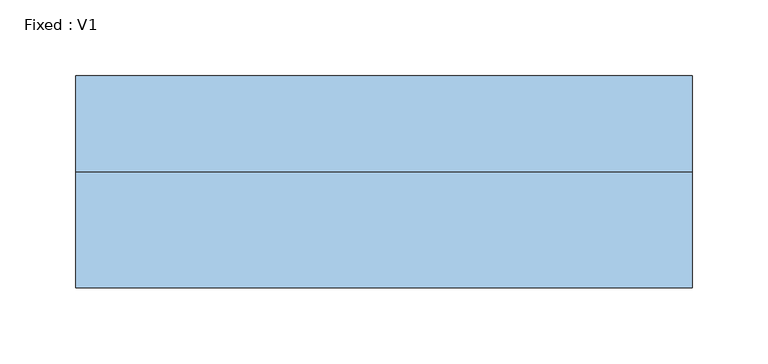
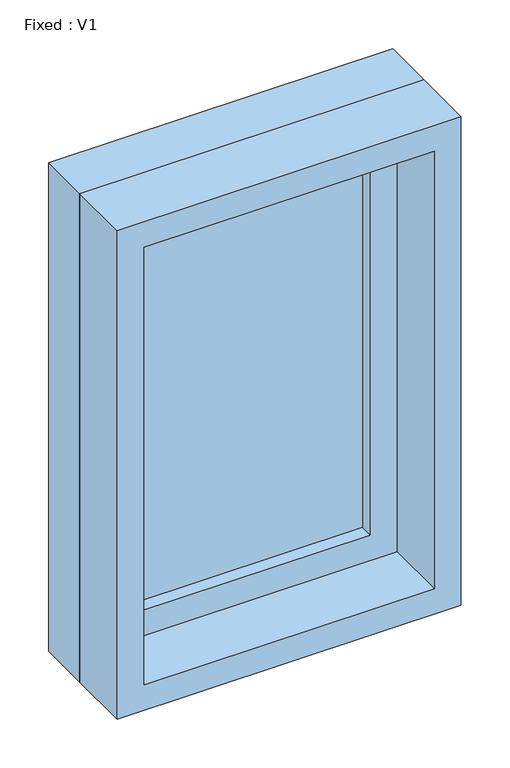
"""IFC4 building model written with IfcOpenShell, lengths in millimetres: window geometry, Fixed : V1."""

from ifc_helpers import new_model, si_unit, frame, origin, place, context, project, spatial, polyline, outline, extrude, source, transform, mapped, element, save


def fixed_v1_ea0d36c9(model_context):
    return source(origin(), model_context, "Body", "SweptSolid", [
        extrude(outline(polyline([(101.6, 22.225), (-177.8, 22.225), (-177.8, 34.925), (101.6, 34.925), (101.6, 22.225)])), frame((0.0, 0.0, 977.9), z_axis=(0.0, 0.0, 1.0), x_axis=(1.0, 0.0, 0.0)), (0.0, 0.0, 1.0), 482.6),
        extrude(outline(polyline([(1504.95, -222.25), (933.45, -222.25), (933.45, 146.05), (1504.95, 146.05), (1504.95, -222.25)]), holes=[polyline([(1460.5, -177.8), (1460.5, 101.6), (977.9, 101.6), (977.9, -177.8), (1460.5, -177.8)])]), frame((0.0, 6.35, 0.0), z_axis=(0.0, 1.0, 0.0), x_axis=(0.0, 0.0, 1.0)), (0.0, 0.0, 1.0), 44.45),
        extrude(outline(polyline([(1524.0, -241.3), (914.4, -241.3), (914.4, 165.1), (1524.0, 165.1), (1524.0, -241.3)]), holes=[polyline([(1492.25, -209.55), (1492.25, 133.35), (946.15, 133.35), (946.15, -209.55), (1492.25, -209.55)])]), frame((0.0, -69.85, 0.0), z_axis=(0.0, 1.0, 0.0), x_axis=(0.0, 0.0, 1.0)), (0.0, 0.0, 1.0), 76.2),
        extrude(outline(polyline([(1524.0, 165.1), (1524.0, -241.3), (914.4, -241.3), (914.4, 165.1), (1524.0, 165.1)]), holes=[polyline([(1504.95, 146.05), (933.45, 146.05), (933.45, -222.25), (1504.95, -222.25), (1504.95, 146.05)])]), frame((0.0, 6.35, 0.0), z_axis=(0.0, 1.0, 0.0), x_axis=(0.0, 0.0, 1.0)), (0.0, 0.0, 1.0), 63.5),
    ])


if __name__ == "__main__":
    model = new_model("IFC4")
    model_context = context("Model", 3, world=origin())
    ifc_project = project(units=[si_unit("LENGTHUNIT", "METRE", prefix="MILLI")], contexts=[model_context])
    site = spatial("IfcSite", under=ifc_project)
    building = spatial("IfcBuilding", under=site)
    placement = place(None, origin())
    fixed_v1_shape = fixed_v1_ea0d36c9(model_context)
    element("IfcWindow", 1, ObjectType="Fixed : V1", at=placement, inside=building, context=model_context, shape_type="MappedRepresentation", body=[
        mapped(fixed_v1_shape, transform((0.0, 0.0, 0.0), x_axis=(1.0, 0.0, 0.0), y_axis=(0.0, 1.0, 0.0), z_axis=(0.0, 0.0, 1.0))),
    ])
    save(model, "model.ifc")

# Revit data of these elements
# Type "Fixed : V1"
#   Type Mark = "V1"
#   Construction Type Id = "GSP4R"
#   Assembly Code = "B2020100"
#   Analytic Construction = "1/8 in Pilkington single glazing"
#   Visual Light Transmittance = 0.9
#   Solar Heat Gain Coefficient = 0.78
#   Heat Transfer Coefficient (U) = 3.6886 W/(m²·K)
#   Height = 609.6 mm
#   Default Sill Height = 914.4 mm
#   Width = 406.4 mm
#   Window Inset = 19.05 mm
#   Glass Pane Material = Glass
#   Sash Material = Sash
#   Wall Closure = (empty or 0)
# Element 1 (IfcWindow, "Fixed : V1")
#   Materials on its faces: "Sash", "Glass"
# Materials
#   "Glass": class "Glass", colour RGB 140 218 255, transparency 0.75, Description = "Soda Lime Glass", Cost = 0
#   "Sash": class "Wood", colour RGB 224 178 126, transparency 0
